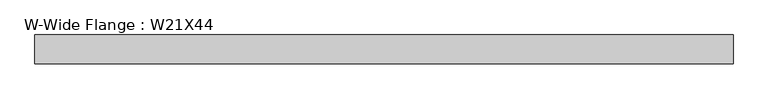
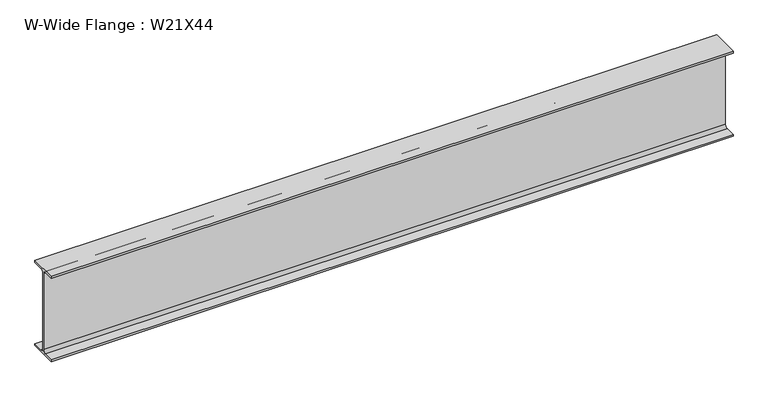
"""IFC4 building model written with IfcOpenShell, lengths in millimetres: beam geometry, W-Wide Flange : W21X44."""

from ifc_helpers import new_model, si_unit, point, frame, frame_2d, origin, place, context, project, spatial, polyline, circle_curve, trimmed, segment, composite_curve, outline, extrude, source, transform, mapped, element, save


def w_wide_flange_w21x44_85607f17(model_context):
    return source(origin(), model_context, "Body", "SweptSolid", [
        extrude(outline(composite_curve([segment(polyline([(82.55, -251.46), (82.55, -262.89), (-82.55, -262.89), (-82.55, -251.46), (-21.59, -251.46)]), True, "CONTINUOUS"), segment(trimmed(circle_curve(frame_2d((-21.59, -234.315)), 17.145), [point((-21.59, -251.46))], [point((-4.445, -234.315))], True, "CARTESIAN"), True, "CONTINUOUS"), segment(polyline([(-4.445, -234.315), (-4.445, 234.315)]), True, "CONTINUOUS"), segment(trimmed(circle_curve(frame_2d((-21.59, 234.315)), 17.145), [point((-4.445, 234.315))], [point((-21.59, 251.46))], True, "CARTESIAN"), True, "CONTINUOUS"), segment(polyline([(-21.59, 251.46), (-82.55, 251.46), (-82.55, 262.89), (82.55, 262.89), (82.55, 251.46), (21.59, 251.46)]), True, "CONTINUOUS"), segment(trimmed(circle_curve(frame_2d((21.59, 234.315)), 17.145), [point((21.59, 251.46))], [point((4.445, 234.315))], True, "CARTESIAN"), True, "CONTINUOUS"), segment(polyline([(4.445, 234.315), (4.445, -234.315)]), True, "CONTINUOUS"), segment(trimmed(circle_curve(frame_2d((21.59, -234.315)), 17.145), [point((4.445, -234.315))], [point((21.59, -251.46))], True, "CARTESIAN"), True, "CONTINUOUS"), segment(polyline([(21.59, -251.46), (82.55, -251.46)]), True, "CONTINUOUS")], self_intersect=False)), frame((-2039.805346, 0.0, 0.0), z_axis=(1.0, 0.0, 0.0), x_axis=(0.0, 1.0, 0.0)), (0.0, 0.0, 1.0), 3975.470692),
    ])


if __name__ == "__main__":
    model = new_model("IFC4")
    model_context = context("Model", 3, world=origin())
    ifc_project = project(units=[si_unit("LENGTHUNIT", "METRE", prefix="MILLI")], contexts=[model_context])
    site = spatial("IfcSite", under=ifc_project)
    building = spatial("IfcBuilding", under=site)
    placement = place(None, origin())
    w_wide_flange_w21x44_shape = w_wide_flange_w21x44_85607f17(model_context)
    element("IfcBeam", 1, ObjectType="W-Wide Flange : W21X44", at=placement, inside=building, context=model_context, shape_type="MappedRepresentation", body=[
        mapped(w_wide_flange_w21x44_shape, transform((0.0, 0.0, 0.0), x_axis=(1.0, 0.0, 0.0), y_axis=(0.0, 1.0, 0.0), z_axis=(0.0, 0.0, 1.0))),
    ])
    save(model, "model.ifc")

# Revit data of these elements
# Type "W-Wide Flange : W21X44"
#   Assembly Code = "B10"
#   W = 44
#   Start Extension Calculation [instance default] = 10' - 0"
#   Start Extension [instance default] = -0' - 0 1/2"
#   End Extension Calculation [instance default] = 10' - 0"
#   End Extension [instance default] = -0' - 0 1/2"
#   Length [instance default] = 5' - 0"
#   bf = 0' - 6 1/2"
#   d = 1' - 8.7"
#   k = 0' - 1 1/8"
#   k2 = 0' - 0.675"
#   tf = 0' - 0.45"
#   tw = 0' - 0.35"
#   A = 0.0902778 SF
#   Beam Material [instance default] = Metal - Steel - ASTM A992
# Element 1 (IfcBeam, "W-Wide Flange : W21X44")
#   Materials on its faces: "Metal - Steel - ASTM A992"
# Materials
#   "Metal - Steel - ASTM A992": class "Metal", colour RGB 128 0 0, transparency 0
